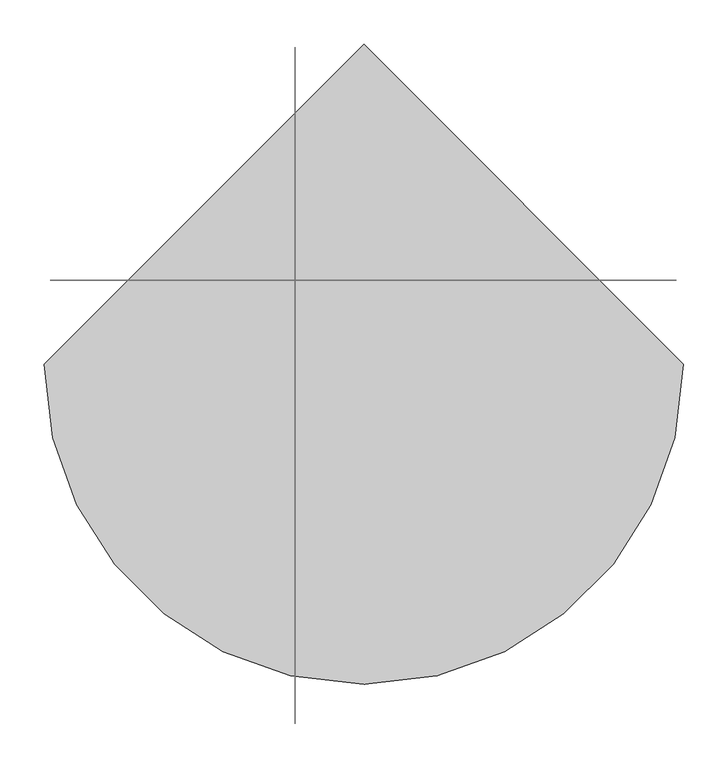
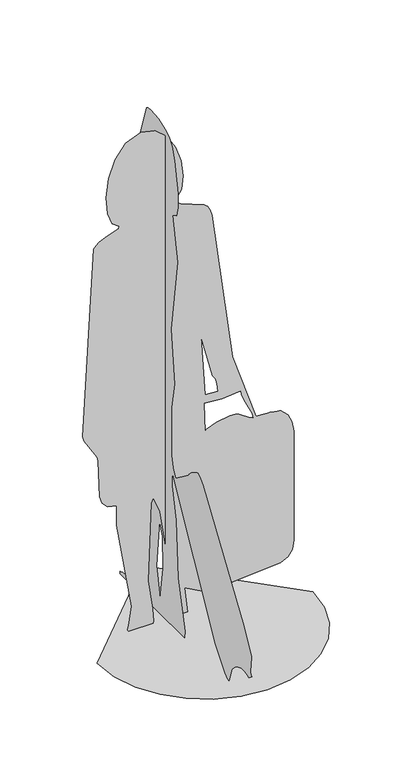
"""IFC4 building model written with IfcOpenShell, lengths in millimetres: proxy geometry, cathy 26654 : cathy 26654."""

import ifcopenshell
import ifcopenshell.guid

model = None  # the IFC model being written
_history = None  # IfcOwnerHistory: only IFC2X3 demands one
_inside = {}  # id of a spatial element -> (the spatial element, [elements in it])
_under = {}  # id of a project, library or spatial element -> (it, [spatial elements below it])
_declared = {}  # id of a project -> (the project, [libraries it declares])
_typed = {}  # id of a type object -> (the type object, [elements of that type])
_made_of = {}  # id of a material, layer set ... -> (it, [elements and type objects made of it])


def new_model(schema):
    """Start an empty IFC model of exactly this schema.

    Asked for "IFC4X3", IfcOpenShell would pick the latest addendum, in which some entities
    have other attributes; the version numbers below select the first issue.
    IFC2X3 requires an IfcOwnerHistory on every rooted entity: one is made here for all.
    """
    global model, _history
    if schema == "IFC4X3":
        model = ifcopenshell.file(schema_version=(4, 3, 0, 0))
    else:
        model = ifcopenshell.file(schema=schema)
    _inside.clear()
    _under.clear()
    _declared.clear()
    _typed.clear()
    _made_of.clear()
    _history = None
    if model.schema == "IFC2X3":
        org = make("IfcOrganization", Name="unknown")
        user = make(
            "IfcPersonAndOrganization",
            ThePerson=make("IfcPerson", FamilyName="unknown"),
            TheOrganization=org,
        )
        app = make(
            "IfcApplication",
            ApplicationDeveloper=org,
            Version="unknown",
            ApplicationFullName="unknown",
            ApplicationIdentifier="unknown",
        )
        _history = make(
            "IfcOwnerHistory",
            OwningUser=user,
            OwningApplication=app,
            ChangeAction="ADDED",
            CreationDate=0,
        )
    return model


def make(cls, **values):
    """One entity of the class cls with the attributes given. An attribute that is None is left unset."""
    return model.create_entity(
        cls, **{name: value for name, value in values.items() if value is not None}
    )


def rooted(cls, **values):
    """An entity with a GlobalId (a new one), such as an element, a storey or a relation."""
    return make(cls, GlobalId=ifcopenshell.guid.new(), OwnerHistory=_history, **values)


def si_unit(unit_type, name, prefix=None):
    """IfcSIUnit, for example si_unit("LENGTHUNIT", "METRE", prefix="MILLI")."""
    return make("IfcSIUnit", UnitType=unit_type, Prefix=prefix, Name=name)


def assignment(units):
    """IfcUnitAssignment: the units of a project."""
    return None if units is None else make("IfcUnitAssignment", Units=units)


def point(xyz):
    """IfcCartesianPoint."""
    return None if xyz is None else make("IfcCartesianPoint", Coordinates=xyz)


def direction(xyz):
    """IfcDirection."""
    return None if xyz is None else make("IfcDirection", DirectionRatios=xyz)


def frame(location, z_axis=None, x_axis=None):
    """IfcAxis2Placement3D, a coordinate frame: its origin and axes. An axis left out is left unset."""
    return make(
        "IfcAxis2Placement3D",
        Location=point(location),
        Axis=direction(z_axis),
        RefDirection=direction(x_axis),
    )


def origin():
    """The frame at (0, 0, 0) with its axes left unset."""
    return frame((0.0, 0.0, 0.0))


def place(relative_to, where):
    """IfcLocalPlacement: puts the frame where relative to a parent placement (None: the world)."""
    return make(
        "IfcLocalPlacement", PlacementRelTo=relative_to, RelativePlacement=where
    )


def context(
    kind, dimensions, precision=None, world=None, true_north=None, identifier=None
):
    """IfcGeometricRepresentationContext, for example the 3D "Model" context."""
    return make(
        "IfcGeometricRepresentationContext",
        ContextIdentifier=identifier,
        ContextType=kind,
        CoordinateSpaceDimension=dimensions,
        Precision=precision,
        WorldCoordinateSystem=world,
        TrueNorth=true_north,
    )


def project(units=None, contexts=None):
    """IfcProject with its units and contexts."""
    return rooted(
        "IfcProject",
        Name="project",
        RepresentationContexts=contexts,
        UnitsInContext=assignment(units),
    )


def spatial(cls, under=None, at=None, **own):
    """A site, building, storey or space (cls), placed at a placement, below another one or the project."""
    s = rooted(cls, ObjectPlacement=at, **own)
    if under is not None:
        _under.setdefault(under.id(), (under, []))[1].append(s)
    return s


def point_list(points):
    """IfcCartesianPointList2D or 3D."""
    cls = (
        "IfcCartesianPointList2D" if len(points[0]) == 2 else "IfcCartesianPointList3D"
    )
    return make(cls, CoordList=points)


def triangles(points, corners, closed=None, point_numbers=None):
    """IfcTriangulatedFaceSet: each triangle names its three corners, points numbered from 1."""
    return make(
        "IfcTriangulatedFaceSet",
        Coordinates=point_list(points),
        Closed=closed,
        CoordIndex=corners,
        PnIndex=point_numbers,
    )


def shape(context_of_items, identifier, shape_type, items):
    """IfcShapeRepresentation: the items that make up one representation, for example the "Body"."""
    return make(
        "IfcShapeRepresentation",
        ContextOfItems=context_of_items,
        RepresentationIdentifier=identifier,
        RepresentationType=shape_type,
        Items=items,
    )


def source(mapping_origin, context_of_items, identifier, shape_type, items):
    """IfcRepresentationMap: a shape defined once, which mapped items show again and again."""
    return make(
        "IfcRepresentationMap",
        MappingOrigin=mapping_origin,
        MappedRepresentation=shape(context_of_items, identifier, shape_type, items),
    )


def transform(
    local_origin,
    x_axis=None,
    y_axis=None,
    z_axis=None,
    scale=None,
    scale2=None,
    scale3=None,
    uniform=True,
):
    """IfcCartesianTransformationOperator3D, or its non-uniform kind. x_axis, y_axis, z_axis: its Axis1, 2, 3."""
    if uniform:
        return make(
            "IfcCartesianTransformationOperator3D",
            Axis1=direction(x_axis),
            Axis2=direction(y_axis),
            LocalOrigin=point(local_origin),
            Scale=scale,
            Axis3=direction(z_axis),
        )
    return make(
        "IfcCartesianTransformationOperator3DnonUniform",
        Axis1=direction(x_axis),
        Axis2=direction(y_axis),
        LocalOrigin=point(local_origin),
        Scale=scale,
        Axis3=direction(z_axis),
        Scale2=scale2,
        Scale3=scale3,
    )


def mapped(mapping_source, mapping_target):
    """IfcMappedItem: shows the shape of a source again, moved by a transform."""
    return make(
        "IfcMappedItem", MappingSource=mapping_source, MappingTarget=mapping_target
    )


def made_of(thing, what):
    """Note that an element or type object is made of a material, layer set ...; save() writes the relation."""
    if what is not None:
        _made_of.setdefault(what.id(), (what, []))[1].append(thing)
    return thing


def element(
    cls,
    number,
    at=None,
    inside=None,
    cuts=None,
    type_object=None,
    material=None,
    context=None,
    identifier="Body",
    shape_type=None,
    held_by="IfcProductDefinitionShape",
    body=None,
    shapes=None,
    **own,
):
    """One element of the class cls, such as IfcWall. Its Tag is "e" and its number.

    at: its placement. inside: the storey or other place that contains it. cuts: it is an
    opening in that element (IfcRelVoidsElement). A single representation is given by context,
    identifier, shape_type and body (its items); several are given by shapes. held_by: the class
    of the entity that holds the representations. save() writes the other relations.
    """
    e = rooted(cls, Tag="e%d" % number, ObjectPlacement=at, **own)
    if body is not None:
        shapes = [shape(context, identifier, shape_type, body)]
    if shapes is not None:
        e.Representation = make(held_by, Representations=shapes)
    if inside is not None:
        _inside.setdefault(inside.id(), (inside, []))[1].append(e)
    if cuts is not None:
        rooted(
            "IfcRelVoidsElement", RelatingBuildingElement=cuts, RelatedOpeningElement=e
        )
    if type_object is not None:
        _typed.setdefault(type_object.id(), (type_object, []))[1].append(e)
    return made_of(e, material)


def aggregate(whole, parts):
    """IfcRelAggregates: a whole, such as a stair, and the parts it consists of."""
    return rooted("IfcRelAggregates", RelatingObject=whole, RelatedObjects=parts)


def save(model, path):
    """Write the relations noted so far, then the file.

    IfcRelAggregates (storeys below a building ...), IfcRelContainedInSpatialStructure (elements
    in a storey), IfcRelDefinesByType, IfcRelAssociatesMaterial and IfcRelDeclares: one each for
    every whole, place, type object, material and project.
    """
    for whole, parts in _under.values():
        aggregate(whole, parts)
    for where, things in _inside.values():
        rooted(
            "IfcRelContainedInSpatialStructure",
            RelatedElements=things,
            RelatingStructure=where,
        )
    for kind, things in _typed.values():
        rooted("IfcRelDefinesByType", RelatedObjects=things, RelatingType=kind)
    for what, things in _made_of.values():
        rooted("IfcRelAssociatesMaterial", RelatedObjects=things, RelatingMaterial=what)
    for by, libraries in _declared.values():
        rooted("IfcRelDeclares", RelatingContext=by, RelatedDefinitions=libraries)
    model.write(path)


def entourage_878ef173(model_context):
    return source(origin(), model_context, "Body", "Tessellation", [
        triangles([(53.8898383, 117.4603358, 747.7914923), (98.2196679, 117.4603358, 744.8361494), (95.1081209, 117.4603176, 773.4306976), (89.3746228, 117.4603176, 791.5245787), (80.4877198, 117.4603176, 806.8979136), (42.0685486, 117.4603086, 957.6191643), (111.0217117, 117.4603449, 714.2722446), (50.9345318, 117.4603358, 718.2382816), (53.8898429, 117.4603449, 617.7574236), (59.3183088, 117.4603449, 623.2589773), (93.5172206, 117.4603449, 636.2914667), (138.3303101, 117.4603449, 644.4038349), (157.0264436, 117.4603449, 643.7551826), (169.1473063, 117.4603449, 638.4446783), (200.5938788, 117.4603449, 617.4117325), (207.9951349, 117.4603449, 613.0218115), (213.5514273, 117.4603449, 610.0099314), (216.4324106, 117.4603449, 608.8914677), (214.1224317, 117.4603449, 624.6304779), (191.1442376, 117.4603449, 672.8652517), (182.9985683, 117.4603449, 688.9846167), (177.0412648, 117.4603449, 704.9755011), (174.7312677, 117.4603449, 720.7485209), (-201.8995404, 117.4604085, 0.0), (-204.1571242, 117.4604085, 3.9497842), (-204.9442855, 117.4604085, 7.6373274), (-204.6662138, 117.4604085, 10.9642256), (-203.7279898, 117.4604085, 13.8318444), (-202.5349122, 117.4604085, 16.1416667), (-201.4920253, 117.4604085, 17.7951722), (-201.0044824, 117.4604085, 18.6940715), (-190.828977, 117.4603994, 85.6587976), (-242.182692, 117.460354, 390.4929889), (-241.6421545, 117.4603449, 458.1701806), (-271.5639473, 117.4603449, 465.087818), (-289.7425615, 117.4603449, 483.6791977), (-298.9889993, 117.4603449, 510.7019305), (-302.8727739, 117.4603176, 638.2599512), (-307.2949422, 117.4603176, 654.1493883), (-350.722742, 117.4603176, 724.6059889), (-355.1449648, 117.4603176, 742.1577518), (-318.2957969, 117.460245, 1393.2515854), (-310.2569707, 117.460245, 1402.8329773), (-299.7625713, 117.460245, 1411.0185242), (-287.5347566, 117.460245, 1417.9618504), (-274.2955575, 117.460245, 1423.8161442), (-260.7672771, 117.460245, 1428.7353207), (-247.6718555, 117.460245, 1432.8724228), (-235.7315414, 117.460245, 1436.3809296), (-232.7762167, 117.4602359, 1445.2468128), (-257.0988964, 117.4602359, 1461.5501781), (-272.1356057, 117.4602177, 1503.7727463), (-276.4824334, 117.4602177, 1561.8838795), (-268.7355044, 117.4602177, 1625.85294), (-247.4909617, 117.4602086, 1685.6494354), (-211.3448214, 117.4601905, 1731.241856), (-158.8932265, 117.4601905, 1752.6), (-111.9791842, 117.4602086, 1741.2460419), (-73.5043479, 117.4602177, 1707.6616093), (-44.4949449, 117.4602177, 1659.4346111), (-25.9771685, 117.4602177, 1604.1516483), (-18.9772346, 117.4602359, 1549.4009205), (-24.5213525, 117.460245, 1502.7694645), (-43.6357222, 117.460245, 1471.8447533), (-41.3971643, 117.460245, 1464.7698944), (-35.6109395, 117.460245, 1458.4332172), (-27.6712375, 117.460245, 1452.9626209), (51.276435, 117.460245, 1421.2944958), (57.2815917, 117.460245, 1416.9136585), (62.600167, 117.460245, 1411.6523518), (67.2046597, 117.460245, 1405.3326794), (71.0676189, 117.460245, 1397.7771812), (78.5116503, 117.460254, 1375.7985809), (147.1776171, 117.4603176, 850.6698057), (225.2983847, 117.4603449, 611.8468105), (275.5388137, 117.460354, 608.9837222), (309.4108014, 117.460354, 601.3092633), (332.2617685, 117.4603721, 580.586255), (345.871948, 117.4603721, 550.2653586), (352.0216816, 117.4603721, 513.7975628), (353.4933941, 117.4604176, 128.4620444), (346.9371809, 117.4604176, 99.2247937), (332.6279889, 117.4604176, 77.1089652), (308.0473672, 117.4604176, 65.1126907), (90.3187149, 117.4604176, 47.8453172), (48.0056181, 117.4604176, 54.0576651), (-14.0824787, 117.4603994, 88.7552838), (-4.1152214, 117.4604176, 0.0), (-74.9051435, 117.4604176, 0.0), (-62.2911333, 117.4603994, 156.8197702), (-96.4066154, 117.4603721, 387.4205747), (-115.2693994, 117.460354, 437.4783113), (-119.5504426, 117.460354, 442.4700125), (-126.1975024, 117.460354, 426.9860739), (-137.0054909, 117.4603994, 156.8197702), (-121.113147, 117.4603994, 51.6135511), (-117.2149747, 117.4604085, 8.0698619), (-119.7951406, 117.4604085, 0.0), (-77.8997872, 135.0692083, 282.8198191), (-77.8998054, 130.3114773, 172.9542868), (-77.8998054, 152.666935, 33.5277909), (-77.8997963, 152.9641916, 69.4067782), (-77.8997963, 169.5678293, 157.0970425), (-77.8997872, 150.7276729, 328.1361483), (-77.8998145, 3.0163209, 25.7191991), (-77.8998054, 45.3518648, 189.0513784), (-77.8997963, 55.7880146, 386.7806791), (-77.8997963, 80.3276914, 494.488567), (-77.8997872, 80.5199489, 517.4922137), (-77.8997872, 76.8446373, 540.9191631), (-77.8998145, -171.7708925, 87.0856001), (-77.8998145, -227.9932601, 18.8921949), (-77.8998236, -243.0883417, 6.7222562), (-77.8998236, -252.4887126, 5.452254), (-77.8998145, -269.9436974, 56.8931116), (-77.8998145, -279.0118393, 68.4347354), (-77.8998236, -291.5888515, 78.625724), (-77.8998236, -306.5133039, 86.7939936), (-77.8998236, -322.6234397, 92.2677329), (-77.8998236, -338.7579563, 94.3743994), (-77.8998236, -353.7550424, 92.4425951), (-77.8998327, -366.4532135, 85.8000045), (-77.8998327, -384.1851617, 100.5765735), (-77.8998327, -379.3155098, 104.3952085), (-77.8998327, -377.4683842, 114.2298371), (-77.8998236, -381.8249496, 165.1035306), (-77.8998236, -381.2298552, 168.5488871), (-77.8998145, -338.4702559, 250.651234), (-77.8997963, -99.3683079, 604.619163), (-77.8997963, -81.9905895, 622.8976622), (-77.8997963, -71.65085, 630.1974346), (-77.8997872, -65.9631884, 629.1904467), (-77.8997963, -34.7905, 610.2242352), (-77.8997963, -19.0469808, 595.6349367), (-77.8997963, -17.7255782, 591.1596285), (-77.8997963, 56.157428, 535.0085137), (-77.8997963, 58.1476771, 537.2532895), (-77.8997872, 66.8439441, 552.4633713), (-77.8997872, 72.0572114, 563.5967397), (-77.8997872, 76.8521041, 575.860853), (-77.8997872, 80.4822059, 588.3398515), (-77.8997782, 82.2011599, 600.1177663), (-77.8997782, 81.1851063, 771.341581), (-77.8997782, 63.9151076, 863.048992), (-77.8997691, 84.6023578, 1046.8329048), (-77.8997691, 47.4761219, 1306.3470062), (-77.8997691, 76.8445827, 1454.1129868), (-77.8997691, 53.8794874, 1467.406216), (-77.8997691, 43.4152415, 1502.0613682), (-77.8997691, 43.0932317, 1550.2417122), (-77.8997509, 63.441213, 1655.8304707), (-77.89976, 79.3938912, 1697.5648418), (-77.8997509, 96.0541751, 1721.476609), (-77.8997509, 113.8033461, 1732.016082), (-77.8997509, 158.8977684, 1746.5525494), (-77.8997418, 202.5220496, 1750.8739426), (-77.8997418, 218.4334876, 1748.6439915), (-77.8997418, 227.5582395, 1743.1885105), (-77.8997509, 274.573284, 1600.1668625), (-77.8997418, 278.9162601, 1559.8313885), (-77.8997509, 274.1262909, 1527.2763988), (-77.8997509, 257.1190804, 1507.3087223), (-77.8997509, 224.7027815, 1486.3441589), (-77.8997509, 208.3494555, 1458.8658943), (-77.89976, 210.3774568, 1428.4683311), (-77.89976, 225.4879443, 1396.3826443), (-77.89976, 296.3251358, 1302.3062645), (-77.89976, 310.7764157, 1275.7776512), (-77.8997691, 316.9745112, 1010.797677), (-77.8997691, 316.2255017, 1004.9043594), (-77.8997782, 295.5383015, 481.8127419), (-77.8997782, 293.46688, 480.3784181), (-77.8997782, 269.2362369, 455.7556841), (-77.8997782, 264.2245697, 447.8189229), (-77.8997782, 261.6443493, 440.3457962), (-77.8997872, 237.1922808, 202.61841), (-77.8997872, 242.132259, 157.050352), (-77.8997872, 253.7944106, 116.4614324), (-77.8997872, 322.1361875, 23.7382494), (-77.8997872, 325.7640547, 23.3657181), (-77.8997872, 333.8459015, 21.7296988), (-77.8997872, 344.6726026, 19.2407246), (-77.8997872, 356.5347055, 16.3091608), (-77.8997872, 367.7233758, 13.3450226), (-77.8997782, 376.529052, 10.7590158), (-77.8997782, 381.2426087, 8.961618), (-77.8997782, 381.1268818, 8.1774101), (-77.8997782, 381.0535578, 7.1637053), (-77.8997782, 381.015624, 5.9590209), (-77.8997782, 381.0058136, 4.6018718), (-77.8997782, 381.0171501, 3.1304315), (-77.8997782, 381.0423666, 1.583731), (-77.8997782, 381.0743777, 0.0001143), (-77.8998145, 6.2281815, 0.0001143), (-361.7310817, 22.4542549, 0.0001143), (-352.1680753, -60.4305955, 0.0001143), (-324.9328191, -136.5470796, 0.0002286), (-282.2059939, -203.7143642, 0.0001143), (-226.1686077, -259.7518049, 0.0001143), (-159.0012504, -302.4785029, 0.0001143), (-82.8847755, -329.7138136, 0.0001143), (6.66e-05, -339.2768563, 0.0001143), (82.8849208, -329.7138863, 0.0001143), (159.0013958, -302.4785574, 0.0002286), (226.1686985, -259.7517323, 0.0001143), (282.2061938, -203.7143824, 0.0001143), (324.9328554, -136.5470251, 0.0001143), (352.1681479, -60.4305456, 0.0001143), (361.7311907, 22.4542844, 0.0002286), (3.3e-06, 384.1853797, 0.0001143)], [[1, 2, 8], [34, 1, 8], [34, 8, 9], [87, 88, 89], [87, 89, 90], [7, 8, 2], [97, 98, 24], [96, 97, 24], [96, 24, 25], [96, 25, 26], [96, 26, 27], [96, 27, 28], [96, 28, 29], [96, 29, 30], [96, 30, 31], [96, 31, 32], [95, 96, 32], [95, 32, 33], [95, 33, 34], [94, 95, 34], [93, 94, 34], [93, 34, 9], [92, 93, 9], [1, 34, 35], [1, 35, 36], [1, 36, 37], [1, 37, 38], [1, 38, 39], [6, 1, 39], [6, 39, 40], [6, 40, 41], [6, 41, 42], [6, 42, 43], [6, 43, 44], [6, 44, 45], [6, 45, 46], [6, 46, 47], [6, 47, 48], [6, 48, 49], [91, 92, 9], [6, 49, 50], [7, 2, 3], [23, 7, 3], [50, 51, 52], [56, 57, 58], [56, 58, 59], [55, 56, 59], [55, 59, 60], [54, 55, 60], [54, 60, 61], [53, 54, 61], [53, 61, 62], [52, 53, 62], [50, 52, 62], [50, 62, 63], [50, 63, 64], [6, 50, 64], [6, 64, 65], [6, 65, 66], [6, 66, 67], [6, 67, 68], [6, 68, 69], [6, 69, 70], [6, 70, 71], [6, 71, 72], [6, 72, 73], [5, 6, 73], [5, 73, 74], [4, 5, 74], [3, 4, 74], [23, 3, 74], [23, 74, 75], [22, 23, 75], [21, 22, 75], [20, 21, 75], [19, 20, 75], [18, 19, 75], [90, 91, 9], [87, 90, 9], [86, 87, 9], [85, 86, 9], [84, 85, 9], [83, 84, 9], [82, 83, 9], [81, 82, 9], [80, 81, 9], [79, 80, 9], [78, 79, 9], [77, 78, 9], [18, 75, 76], [12, 13, 14], [11, 12, 14], [11, 14, 15], [10, 11, 15], [9, 10, 15], [9, 15, 16], [9, 16, 17], [9, 17, 18], [77, 9, 18], [77, 18, 76], [100, 101, 106], [122, 123, 124], [100, 106, 107], [99, 100, 107], [104, 99, 107], [105, 106, 101], [194, 105, 101], [193, 194, 101], [192, 193, 101], [191, 192, 101], [190, 191, 101], [189, 190, 101], [188, 189, 101], [187, 188, 101], [186, 187, 101], [185, 186, 101], [184, 185, 101], [183, 184, 101], [182, 183, 101], [181, 182, 101], [180, 181, 101], [179, 180, 101], [178, 179, 101], [178, 101, 102], [177, 178, 102], [177, 102, 103], [176, 177, 103], [175, 176, 103], [175, 103, 104], [121, 122, 124], [113, 114, 115], [112, 113, 115], [111, 112, 115], [121, 124, 125], [175, 104, 107], [175, 107, 108], [174, 175, 108], [174, 108, 109], [173, 174, 109], [173, 109, 110], [172, 173, 110], [111, 115, 116], [170, 171, 172], [170, 172, 110], [120, 121, 125], [120, 125, 126], [111, 116, 117], [111, 117, 118], [110, 111, 118], [110, 118, 119], [110, 119, 120], [110, 120, 126], [110, 126, 127], [110, 127, 128], [130, 131, 132], [147, 148, 149], [129, 130, 132], [129, 132, 133], [129, 133, 134], [129, 134, 135], [129, 135, 136], [128, 129, 136], [110, 128, 136], [110, 136, 137], [110, 137, 138], [170, 110, 138], [170, 138, 139], [170, 139, 140], [170, 140, 141], [170, 141, 142], [170, 142, 143], [170, 143, 144], [170, 144, 145], [169, 170, 145], [168, 169, 145], [167, 168, 145], [167, 145, 146], [166, 167, 146], [165, 166, 146], [164, 165, 146], [164, 146, 147], [164, 147, 149], [164, 149, 150], [163, 164, 150], [163, 150, 151], [162, 163, 151], [161, 162, 151], [160, 161, 151], [159, 160, 151], [159, 151, 152], [159, 152, 153], [159, 153, 154], [159, 154, 155], [159, 155, 156], [158, 159, 156], [158, 156, 157], [209, 210, 195], [208, 209, 195], [208, 195, 196], [207, 208, 196], [207, 196, 197], [207, 197, 198], [206, 207, 198], [205, 206, 198], [205, 198, 199], [205, 199, 200], [205, 200, 201], [205, 201, 202], [205, 202, 203], [205, 203, 204]], closed=False),
    ])


if __name__ == "__main__":
    model = new_model("IFC4")
    model_context = context("Model", 3, world=origin())
    ifc_project = project(units=[si_unit("LENGTHUNIT", "METRE", prefix="MILLI")], contexts=[model_context])
    site = spatial("IfcSite", under=ifc_project)
    building = spatial("IfcBuilding", under=site)
    placement = place(None, origin())
    entourage_shape = entourage_878ef173(model_context)
    element("IfcBuildingElementProxy", 1, Name="cathy 26654 : cathy 26654", ObjectType="cathy 26654 : cathy 26654", at=placement, inside=building, context=model_context, shape_type="MappedRepresentation", body=[
        mapped(entourage_shape, transform((0.0, 0.0, 0.0), x_axis=(1.0, 0.0, 0.0), y_axis=(0.0, 1.0, 0.0), z_axis=(0.0, 0.0, 1.0))),
    ])
    save(model, "model.ifc")

# Revit data of these elements
# Type "cathy 26654 : cathy 26654"
#   built-in parameter 1005195 = "RPC-8-G1GX-ADPX-7HAL-C"
#   Height = 0
